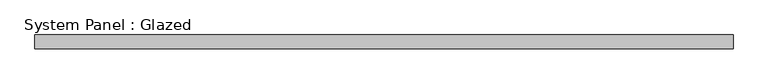
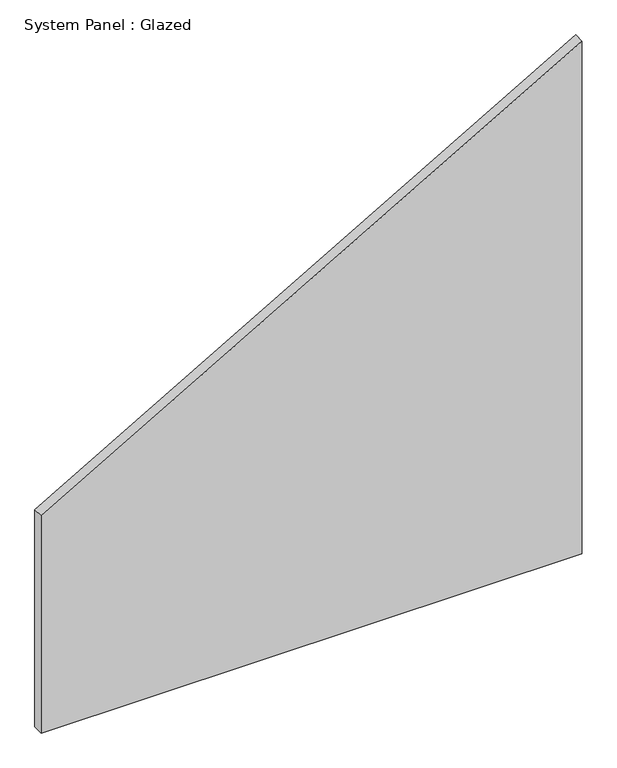
"""IFC4 building model written with IfcOpenShell, lengths in millimetres: plate geometry, System Panel : Glazed."""

from ifc_helpers import new_model, si_unit, frame, origin, place, context, project, spatial, polyline, outline, extrude, source, transform, mapped, element, save


def system_panel_glazed_ad7ef3dc(model_context):
    return source(origin(), model_context, "Body", "SweptSolid", [
        extrude(outline(polyline([(0.0, -626.7857144), (0.0, 626.7857144), (1255.5229345, 626.7857144), (531.7731326, -626.7857144), (0.0, -626.7857144)])), frame((0.0, 24.5, 0.0), z_axis=(0.0, 1.0, 0.0), x_axis=(0.0, 0.0, 1.0)), (0.0, 0.0, 1.0), 25.0),
    ])


if __name__ == "__main__":
    model = new_model("IFC4")
    model_context = context("Model", 3, world=origin())
    ifc_project = project(units=[si_unit("LENGTHUNIT", "METRE", prefix="MILLI")], contexts=[model_context])
    site = spatial("IfcSite", under=ifc_project)
    building = spatial("IfcBuilding", under=site)
    placement = place(None, origin())
    system_panel_glazed_shape = system_panel_glazed_ad7ef3dc(model_context)
    element("IfcPlate", 1, ObjectType="System Panel : Glazed", at=placement, inside=building, context=model_context, shape_type="MappedRepresentation", body=[
        mapped(system_panel_glazed_shape, transform((0.0, 0.0, 0.0), x_axis=(1.0, 0.0, 0.0), y_axis=(0.0, 1.0, 0.0), z_axis=(0.0, 0.0, 1.0))),
    ])
    save(model, "model.ifc")

# Revit data of these elements
# Type "System Panel : Glazed"
#   Construction Type Id = "GSP4R"
#   Analytic Construction = "1/8 in Pilkington single glazing"
#   Visual Light Transmittance = 0.9
#   Solar Heat Gain Coefficient = 0.86
#   Heat Transfer Coefficient (U) = 6.7069 W/(m²·K)
#   Define Thermal Properties by = 1
# Element 1 (IfcPlate, "System Panel : Glazed")
#   Materials on its faces: "Glass"
# Materials
#   "Glass": class "Glass", colour RGB 0 128 192, transparency 0.75, Description = "Soda Lime Glass", Cost = 0
